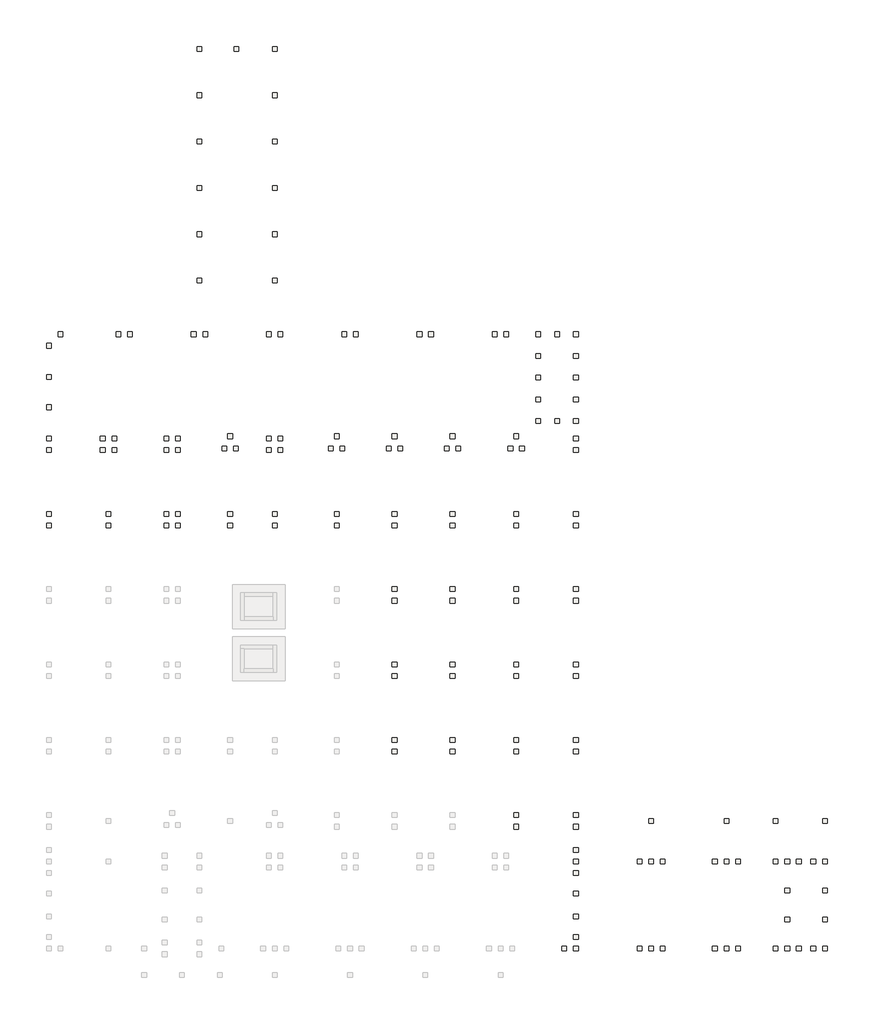
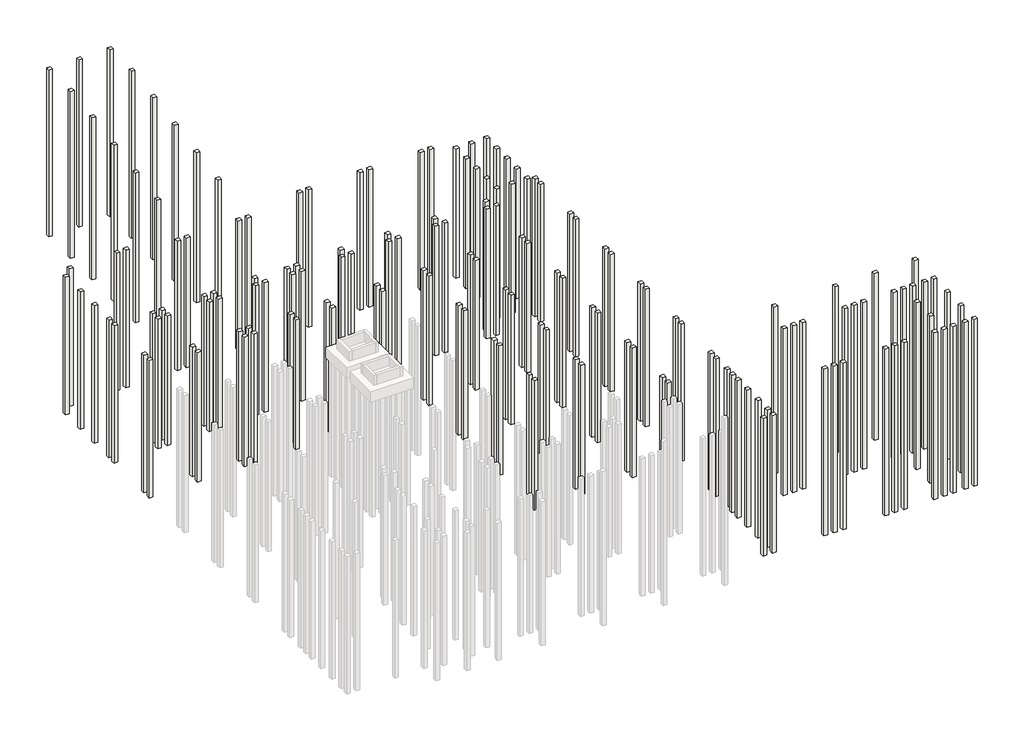
# Not in any storey, part 2 of 2: 160 slabs.
"""IFC4 building model written with IfcOpenShell, lengths in millimetres."""

import ifcopenshell
import ifcopenshell.guid

model = None  # the IFC model being written
_history = None  # IfcOwnerHistory: only IFC2X3 demands one
_inside = {}  # id of a spatial element -> (the spatial element, [elements in it])
_under = {}  # id of a project, library or spatial element -> (it, [spatial elements below it])
_declared = {}  # id of a project -> (the project, [libraries it declares])
_typed = {}  # id of a type object -> (the type object, [elements of that type])
_made_of = {}  # id of a material, layer set ... -> (it, [elements and type objects made of it])


def new_model(schema):
    """Start an empty IFC model of exactly this schema.

    Asked for "IFC4X3", IfcOpenShell would pick the latest addendum, in which some entities
    have other attributes; the version numbers below select the first issue.
    IFC2X3 requires an IfcOwnerHistory on every rooted entity: one is made here for all.
    """
    global model, _history
    if schema == "IFC4X3":
        model = ifcopenshell.file(schema_version=(4, 3, 0, 0))
    else:
        model = ifcopenshell.file(schema=schema)
    _inside.clear()
    _under.clear()
    _declared.clear()
    _typed.clear()
    _made_of.clear()
    _history = None
    if model.schema == "IFC2X3":
        org = make("IfcOrganization", Name="unknown")
        user = make(
            "IfcPersonAndOrganization",
            ThePerson=make("IfcPerson", FamilyName="unknown"),
            TheOrganization=org,
        )
        app = make(
            "IfcApplication",
            ApplicationDeveloper=org,
            Version="unknown",
            ApplicationFullName="unknown",
            ApplicationIdentifier="unknown",
        )
        _history = make(
            "IfcOwnerHistory",
            OwningUser=user,
            OwningApplication=app,
            ChangeAction="ADDED",
            CreationDate=0,
        )
    return model


def make(cls, **values):
    """One entity of the class cls with the attributes given. An attribute that is None is left unset."""
    return model.create_entity(
        cls, **{name: value for name, value in values.items() if value is not None}
    )


def rooted(cls, **values):
    """An entity with a GlobalId (a new one), such as an element, a storey or a relation."""
    return make(cls, GlobalId=ifcopenshell.guid.new(), OwnerHistory=_history, **values)


def si_unit(unit_type, name, prefix=None):
    """IfcSIUnit, for example si_unit("LENGTHUNIT", "METRE", prefix="MILLI")."""
    return make("IfcSIUnit", UnitType=unit_type, Prefix=prefix, Name=name)


def assignment(units):
    """IfcUnitAssignment: the units of a project."""
    return None if units is None else make("IfcUnitAssignment", Units=units)


def point(xyz):
    """IfcCartesianPoint."""
    return None if xyz is None else make("IfcCartesianPoint", Coordinates=xyz)


def direction(xyz):
    """IfcDirection."""
    return None if xyz is None else make("IfcDirection", DirectionRatios=xyz)


def frame(location, z_axis=None, x_axis=None):
    """IfcAxis2Placement3D, a coordinate frame: its origin and axes. An axis left out is left unset."""
    return make(
        "IfcAxis2Placement3D",
        Location=point(location),
        Axis=direction(z_axis),
        RefDirection=direction(x_axis),
    )


def origin():
    """The frame at (0, 0, 0) with its axes left unset."""
    return frame((0.0, 0.0, 0.0))


def place(relative_to, where):
    """IfcLocalPlacement: puts the frame where relative to a parent placement (None: the world)."""
    return make(
        "IfcLocalPlacement", PlacementRelTo=relative_to, RelativePlacement=where
    )


def context(
    kind, dimensions, precision=None, world=None, true_north=None, identifier=None
):
    """IfcGeometricRepresentationContext, for example the 3D "Model" context."""
    return make(
        "IfcGeometricRepresentationContext",
        ContextIdentifier=identifier,
        ContextType=kind,
        CoordinateSpaceDimension=dimensions,
        Precision=precision,
        WorldCoordinateSystem=world,
        TrueNorth=true_north,
    )


def project(units=None, contexts=None):
    """IfcProject with its units and contexts."""
    return rooted(
        "IfcProject",
        Name="project",
        RepresentationContexts=contexts,
        UnitsInContext=assignment(units),
    )


def spatial(cls, under=None, at=None, **own):
    """A site, building, storey or space (cls), placed at a placement, below another one or the project."""
    s = rooted(cls, ObjectPlacement=at, **own)
    if under is not None:
        _under.setdefault(under.id(), (under, []))[1].append(s)
    return s


def polyline(points):
    """IfcPolyline through the points."""
    return make("IfcPolyline", Points=[point(p) for p in points])


def outline(outer, holes=None, kind="AREA"):
    """IfcArbitraryClosedProfileDef: a profile drawn as a closed curve; with holes, ...WithVoids."""
    if holes is None:
        return make("IfcArbitraryClosedProfileDef", ProfileType=kind, OuterCurve=outer)
    return make(
        "IfcArbitraryProfileDefWithVoids",
        ProfileType=kind,
        OuterCurve=outer,
        InnerCurves=holes,
    )


def extrude(swept, where, along, depth):
    """IfcExtrudedAreaSolid: the profile swept, set in the frame where, extruded along a direction by depth."""
    return make(
        "IfcExtrudedAreaSolid",
        SweptArea=swept,
        Position=where,
        ExtrudedDirection=direction(along),
        Depth=depth,
    )


def shape(context_of_items, identifier, shape_type, items):
    """IfcShapeRepresentation: the items that make up one representation, for example the "Body"."""
    return make(
        "IfcShapeRepresentation",
        ContextOfItems=context_of_items,
        RepresentationIdentifier=identifier,
        RepresentationType=shape_type,
        Items=items,
    )


def source(mapping_origin, context_of_items, identifier, shape_type, items):
    """IfcRepresentationMap: a shape defined once, which mapped items show again and again."""
    return make(
        "IfcRepresentationMap",
        MappingOrigin=mapping_origin,
        MappedRepresentation=shape(context_of_items, identifier, shape_type, items),
    )


def transform(
    local_origin,
    x_axis=None,
    y_axis=None,
    z_axis=None,
    scale=None,
    scale2=None,
    scale3=None,
    uniform=True,
):
    """IfcCartesianTransformationOperator3D, or its non-uniform kind. x_axis, y_axis, z_axis: its Axis1, 2, 3."""
    if uniform:
        return make(
            "IfcCartesianTransformationOperator3D",
            Axis1=direction(x_axis),
            Axis2=direction(y_axis),
            LocalOrigin=point(local_origin),
            Scale=scale,
            Axis3=direction(z_axis),
        )
    return make(
        "IfcCartesianTransformationOperator3DnonUniform",
        Axis1=direction(x_axis),
        Axis2=direction(y_axis),
        LocalOrigin=point(local_origin),
        Scale=scale,
        Axis3=direction(z_axis),
        Scale2=scale2,
        Scale3=scale3,
    )


def mapped(mapping_source, mapping_target):
    """IfcMappedItem: shows the shape of a source again, moved by a transform."""
    return make(
        "IfcMappedItem", MappingSource=mapping_source, MappingTarget=mapping_target
    )


def made_of(thing, what):
    """Note that an element or type object is made of a material, layer set ...; save() writes the relation."""
    if what is not None:
        _made_of.setdefault(what.id(), (what, []))[1].append(thing)
    return thing


def element(
    cls,
    number,
    at=None,
    inside=None,
    cuts=None,
    type_object=None,
    material=None,
    context=None,
    identifier="Body",
    shape_type=None,
    held_by="IfcProductDefinitionShape",
    body=None,
    shapes=None,
    **own,
):
    """One element of the class cls, such as IfcWall. Its Tag is "e" and its number.

    at: its placement. inside: the storey or other place that contains it. cuts: it is an
    opening in that element (IfcRelVoidsElement). A single representation is given by context,
    identifier, shape_type and body (its items); several are given by shapes. held_by: the class
    of the entity that holds the representations. save() writes the other relations.
    """
    e = rooted(cls, Tag="e%d" % number, ObjectPlacement=at, **own)
    if body is not None:
        shapes = [shape(context, identifier, shape_type, body)]
    if shapes is not None:
        e.Representation = make(held_by, Representations=shapes)
    if inside is not None:
        _inside.setdefault(inside.id(), (inside, []))[1].append(e)
    if cuts is not None:
        rooted(
            "IfcRelVoidsElement", RelatingBuildingElement=cuts, RelatedOpeningElement=e
        )
    if type_object is not None:
        _typed.setdefault(type_object.id(), (type_object, []))[1].append(e)
    return made_of(e, material)


def aggregate(whole, parts):
    """IfcRelAggregates: a whole, such as a stair, and the parts it consists of."""
    return rooted("IfcRelAggregates", RelatingObject=whole, RelatedObjects=parts)


def save(model, path):
    """Write the relations noted so far, then the file.

    IfcRelAggregates (storeys below a building ...), IfcRelContainedInSpatialStructure (elements
    in a storey), IfcRelDefinesByType, IfcRelAssociatesMaterial and IfcRelDeclares: one each for
    every whole, place, type object, material and project.
    """
    for whole, parts in _under.values():
        aggregate(whole, parts)
    for where, things in _inside.values():
        rooted(
            "IfcRelContainedInSpatialStructure",
            RelatedElements=things,
            RelatingStructure=where,
        )
    for kind, things in _typed.values():
        rooted("IfcRelDefinesByType", RelatedObjects=things, RelatingType=kind)
    for what, things in _made_of.values():
        rooted("IfcRelAssociatesMaterial", RelatedObjects=things, RelatingMaterial=what)
    for by, libraries in _declared.values():
        rooted("IfcRelDeclares", RelatingContext=by, RelatedDefinitions=libraries)
    model.write(path)


def slab_2462c6b3(model_context):
    return source(origin(), model_context, "Body", "SweptSolid", [
        extrude(outline(polyline([(200.0, -200.0), (-200.0, -200.0), (-200.0, 200.0), (200.0, 200.0), (200.0, -200.0)])), frame((0.0, 0.0, -20000.0), z_axis=(0.0, 0.0, 1.0), x_axis=(1.0, 0.0, 0.0)), (0.0, 0.0, 1.0), 14620.0),
    ])


def slab_4eaa82be(model_context):
    return source(origin(), model_context, "Body", "SweptSolid", [
        extrude(outline(polyline([(200.0, -200.0), (-200.0, -200.0), (-200.0, 200.0), (200.0, 200.0), (200.0, -200.0)])), frame((0.0, 0.0, -20000.0), z_axis=(0.0, 0.0, 1.0), x_axis=(1.0, 0.0, 0.0)), (0.0, 0.0, 1.0), 15520.0),
    ])


def slab_c87ae41e(model_context):
    return source(origin(), model_context, "Body", "SweptSolid", [
        extrude(outline(polyline([(200.0, -200.0), (-200.0, -200.0), (-200.0, 200.0), (200.0, 200.0), (200.0, -200.0)])), frame((0.0, 0.0, -20000.0), z_axis=(0.0, 0.0, 1.0), x_axis=(1.0, 0.0, 0.0)), (0.0, 0.0, 1.0), 18830.0),
    ])


def slab_0d914d5e(model_context):
    return source(origin(), model_context, "Body", "SweptSolid", [
        extrude(outline(polyline([(200.0, -200.0), (-200.0, -200.0), (-200.0, 200.0), (200.0, 200.0), (200.0, -200.0)])), frame((0.0, 0.0, -20000.0), z_axis=(0.0, 0.0, 1.0), x_axis=(1.0, 0.0, 0.0)), (0.0, 0.0, 1.0), 18850.0),
    ])


def slab_c32f4c5b(model_context):
    return source(origin(), model_context, "Body", "SweptSolid", [
        extrude(outline(polyline([(200.0, -200.0), (-200.0, -200.0), (-200.0, 200.0), (200.0, 200.0), (200.0, -200.0)])), frame((0.0, 0.0, -20000.0), z_axis=(0.0, 0.0, 1.0), x_axis=(1.0, 0.0, 0.0)), (0.0, 0.0, 1.0), 18290.0),
    ])


def slab_f6128070(model_context):
    return source(origin(), model_context, "Body", "SweptSolid", [
        extrude(outline(polyline([(200.0, -200.0), (-200.0, -200.0), (-200.0, 200.0), (200.0, 200.0), (200.0, -200.0)])), frame((0.0, 0.0, -20000.0), z_axis=(0.0, 0.0, 1.0), x_axis=(1.0, 0.0, 0.0)), (0.0, 0.0, 1.0), 17610.0),
    ])


def slab_f9187350(model_context):
    return source(origin(), model_context, "Body", "SweptSolid", [
        extrude(outline(polyline([(200.0, -200.0), (-200.0, -200.0), (-200.0, 200.0), (200.0, 200.0), (200.0, -200.0)])), frame((0.0, 0.0, -20000.0), z_axis=(0.0, 0.0, 1.0), x_axis=(1.0, 0.0, 0.0)), (0.0, 0.0, 1.0), 16925.0),
    ])


def slab_d279473c(model_context):
    return source(origin(), model_context, "Body", "SweptSolid", [
        extrude(outline(polyline([(200.0, -200.0), (-200.0, -200.0), (-200.0, 200.0), (200.0, 200.0), (200.0, -200.0)])), frame((0.0, 0.0, -20000.0), z_axis=(0.0, 0.0, 1.0), x_axis=(1.0, 0.0, 0.0)), (0.0, 0.0, 1.0), 16250.0),
    ])


model = new_model("IFC4")

# Units and contexts
model_context = context("Model", 3, world=origin())
ifc_project = project(units=[si_unit("LENGTHUNIT", "METRE", prefix="MILLI")], contexts=[model_context])

# Site, building
site = spatial("IfcSite", under=ifc_project)
building = spatial("IfcBuilding", under=site)

# Slabs
placement = place(None, origin())
slab_shape = slab_2462c6b3(model_context)
element("IfcSlab", 1, at=placement, inside=building, context=model_context, shape_type="MappedRepresentation", body=[
    mapped(slab_shape, transform((11650.0, 36500.0, 0.0), x_axis=(1.0, 0.0, 0.0), y_axis=(0.0, 1.0, 0.0), z_axis=(0.0, 0.0, 1.0))),
])
element("IfcSlab", 2, at=placement, inside=building, context=model_context, shape_type="MappedRepresentation", body=[
    mapped(slab_shape, transform((11650.0, 37500.0, 0.0), x_axis=(1.0, 0.0, 0.0), y_axis=(0.0, 1.0, 0.0), z_axis=(0.0, 0.0, 1.0))),
])
element("IfcSlab", 3, at=placement, inside=building, context=model_context, shape_type="MappedRepresentation", body=[
    mapped(slab_shape, transform((22150.0, 36500.0, 0.0), x_axis=(1.0, 0.0, 0.0), y_axis=(0.0, 1.0, 0.0), z_axis=(0.0, 0.0, 1.0))),
])
element("IfcSlab", 4, at=placement, inside=building, context=model_context, shape_type="MappedRepresentation", body=[
    mapped(slab_shape, transform((22150.0, 37500.0, 0.0), x_axis=(1.0, 0.0, 0.0), y_axis=(0.0, 1.0, 0.0), z_axis=(0.0, 0.0, 1.0))),
])
element("IfcSlab", 5, at=placement, inside=building, context=model_context, shape_type="MappedRepresentation", body=[
    mapped(slab_shape, transform((26000.0, 36500.0, 0.0), x_axis=(1.0, 0.0, 0.0), y_axis=(0.0, 1.0, 0.0), z_axis=(0.0, 0.0, 1.0))),
])
element("IfcSlab", 6, at=placement, inside=building, context=model_context, shape_type="MappedRepresentation", body=[
    mapped(slab_shape, transform((26000.0, 37500.0, 0.0), x_axis=(1.0, 0.0, 0.0), y_axis=(0.0, 1.0, 0.0), z_axis=(0.0, 0.0, 1.0))),
])
element("IfcSlab", 7, at=placement, inside=building, context=model_context, shape_type="MappedRepresentation", body=[
    mapped(slab_shape, transform((46850.0, 10500.0, 0.0), x_axis=(1.0, 0.0, 0.0), y_axis=(0.0, 1.0, 0.0), z_axis=(0.0, 0.0, 1.0))),
])
element("IfcSlab", 8, at=placement, inside=building, context=model_context, shape_type="MappedRepresentation", body=[
    mapped(slab_shape, transform((46850.0, 11500.0, 0.0), x_axis=(1.0, 0.0, 0.0), y_axis=(0.0, 1.0, 0.0), z_axis=(0.0, 0.0, 1.0))),
])
element("IfcSlab", 9, at=placement, inside=building, context=model_context, shape_type="MappedRepresentation", body=[
    mapped(slab_shape, transform((17650.0, 36500.0, 0.0), x_axis=(1.0, 0.0, 0.0), y_axis=(0.0, 1.0, 0.0), z_axis=(0.0, 0.0, 1.0))),
])
element("IfcSlab", 10, at=placement, inside=building, context=model_context, shape_type="MappedRepresentation", body=[
    mapped(slab_shape, transform((17650.0, 37500.0, 0.0), x_axis=(1.0, 0.0, 0.0), y_axis=(0.0, 1.0, 0.0), z_axis=(0.0, 0.0, 1.0))),
])
element("IfcSlab", 11, at=placement, inside=building, context=model_context, shape_type="MappedRepresentation", body=[
    mapped(slab_shape, transform((16650.0, 36500.0, 0.0), x_axis=(1.0, 0.0, 0.0), y_axis=(0.0, 1.0, 0.0), z_axis=(0.0, 0.0, 1.0))),
])
element("IfcSlab", 12, at=placement, inside=building, context=model_context, shape_type="MappedRepresentation", body=[
    mapped(slab_shape, transform((16650.0, 37500.0, 0.0), x_axis=(1.0, 0.0, 0.0), y_axis=(0.0, 1.0, 0.0), z_axis=(0.0, 0.0, 1.0))),
])
element("IfcSlab", 13, at=placement, inside=building, context=model_context, shape_type="MappedRepresentation", body=[
    mapped(slab_shape, transform((48755.0, 45500.0, 0.0), x_axis=(1.0, 0.0, 0.0), y_axis=(0.0, 1.0, 0.0), z_axis=(0.0, 0.0, 1.0))),
])
element("IfcSlab", 14, at=placement, inside=building, context=model_context, shape_type="MappedRepresentation", body=[
    mapped(slab_shape, transform((52000.0, 45500.0, 0.0), x_axis=(1.0, 0.0, 0.0), y_axis=(0.0, 1.0, 0.0), z_axis=(0.0, 0.0, 1.0))),
])
element("IfcSlab", 15, at=placement, inside=building, context=model_context, shape_type="MappedRepresentation", body=[
    mapped(slab_shape, transform((52000.0, 53000.0, 0.0), x_axis=(1.0, 0.0, 0.0), y_axis=(0.0, 1.0, 0.0), z_axis=(0.0, 0.0, 1.0))),
])
element("IfcSlab", 16, at=placement, inside=building, context=model_context, shape_type="MappedRepresentation", body=[
    mapped(slab_shape, transform((48755.0, 53000.0, 0.0), x_axis=(1.0, 0.0, 0.0), y_axis=(0.0, 1.0, 0.0), z_axis=(0.0, 0.0, 1.0))),
])
element("IfcSlab", 17, at=placement, inside=building, context=model_context, shape_type="MappedRepresentation", body=[
    mapped(slab_shape, transform((50377.5, 53000.0, 0.0), x_axis=(1.0, 0.0, 0.0), y_axis=(0.0, 1.0, 0.0), z_axis=(0.0, 0.0, 1.0))),
])
element("IfcSlab", 18, at=placement, inside=building, context=model_context, shape_type="MappedRepresentation", body=[
    mapped(slab_shape, transform((50377.5, 45500.0, 0.0), x_axis=(1.0, 0.0, 0.0), y_axis=(0.0, 1.0, 0.0), z_axis=(0.0, 0.0, 1.0))),
])
element("IfcSlab", 19, at=placement, inside=building, context=model_context, shape_type="MappedRepresentation", body=[
    mapped(slab_shape, transform((48755.0, 47375.0, 0.0), x_axis=(1.0, 0.0, 0.0), y_axis=(0.0, 1.0, 0.0), z_axis=(0.0, 0.0, 1.0))),
])
element("IfcSlab", 20, at=placement, inside=building, context=model_context, shape_type="MappedRepresentation", body=[
    mapped(slab_shape, transform((48755.0, 49250.0, 0.0), x_axis=(1.0, 0.0, 0.0), y_axis=(0.0, 1.0, 0.0), z_axis=(0.0, 0.0, 1.0))),
])
element("IfcSlab", 21, at=placement, inside=building, context=model_context, shape_type="MappedRepresentation", body=[
    mapped(slab_shape, transform((48755.0, 51125.0, 0.0), x_axis=(1.0, 0.0, 0.0), y_axis=(0.0, 1.0, 0.0), z_axis=(0.0, 0.0, 1.0))),
])
element("IfcSlab", 22, at=placement, inside=building, context=model_context, shape_type="MappedRepresentation", body=[
    mapped(slab_shape, transform((52000.0, 47375.0, 0.0), x_axis=(1.0, 0.0, 0.0), y_axis=(0.0, 1.0, 0.0), z_axis=(0.0, 0.0, 1.0))),
])
element("IfcSlab", 23, at=placement, inside=building, context=model_context, shape_type="MappedRepresentation", body=[
    mapped(slab_shape, transform((52000.0, 49250.0, 0.0), x_axis=(1.0, 0.0, 0.0), y_axis=(0.0, 1.0, 0.0), z_axis=(0.0, 0.0, 1.0))),
])
element("IfcSlab", 24, at=placement, inside=building, context=model_context, shape_type="MappedRepresentation", body=[
    mapped(slab_shape, transform((52000.0, 51125.0, 0.0), x_axis=(1.0, 0.0, 0.0), y_axis=(0.0, 1.0, 0.0), z_axis=(0.0, 0.0, 1.0))),
])
element("IfcSlab", 25, at=placement, inside=building, context=model_context, shape_type="MappedRepresentation", body=[
    mapped(slab_shape, transform((36350.0, 17000.0, 0.0), x_axis=(1.0, 0.0, 0.0), y_axis=(0.0, 1.0, 0.0), z_axis=(0.0, 0.0, 1.0))),
])
element("IfcSlab", 26, at=placement, inside=building, context=model_context, shape_type="MappedRepresentation", body=[
    mapped(slab_shape, transform((36350.0, 18000.0, 0.0), x_axis=(1.0, 0.0, 0.0), y_axis=(0.0, 1.0, 0.0), z_axis=(0.0, 0.0, 1.0))),
])
element("IfcSlab", 27, at=placement, inside=building, context=model_context, shape_type="MappedRepresentation", body=[
    mapped(slab_shape, transform((41350.0, 17000.0, 0.0), x_axis=(1.0, 0.0, 0.0), y_axis=(0.0, 1.0, 0.0), z_axis=(0.0, 0.0, 1.0))),
])
element("IfcSlab", 28, at=placement, inside=building, context=model_context, shape_type="MappedRepresentation", body=[
    mapped(slab_shape, transform((41350.0, 18000.0, 0.0), x_axis=(1.0, 0.0, 0.0), y_axis=(0.0, 1.0, 0.0), z_axis=(0.0, 0.0, 1.0))),
])
element("IfcSlab", 29, at=placement, inside=building, context=model_context, shape_type="MappedRepresentation", body=[
    mapped(slab_shape, transform((46850.0, 17000.0, 0.0), x_axis=(1.0, 0.0, 0.0), y_axis=(0.0, 1.0, 0.0), z_axis=(0.0, 0.0, 1.0))),
])
element("IfcSlab", 30, at=placement, inside=building, context=model_context, shape_type="MappedRepresentation", body=[
    mapped(slab_shape, transform((46850.0, 18000.0, 0.0), x_axis=(1.0, 0.0, 0.0), y_axis=(0.0, 1.0, 0.0), z_axis=(0.0, 0.0, 1.0))),
])
element("IfcSlab", 31, at=placement, inside=building, context=model_context, shape_type="MappedRepresentation", body=[
    mapped(slab_shape, transform((46850.0, 23500.0, 0.0), x_axis=(1.0, 0.0, 0.0), y_axis=(0.0, 1.0, 0.0), z_axis=(0.0, 0.0, 1.0))),
])
element("IfcSlab", 32, at=placement, inside=building, context=model_context, shape_type="MappedRepresentation", body=[
    mapped(slab_shape, transform((46850.0, 24500.0, 0.0), x_axis=(1.0, 0.0, 0.0), y_axis=(0.0, 1.0, 0.0), z_axis=(0.0, 0.0, 1.0))),
])
element("IfcSlab", 33, at=placement, inside=building, context=model_context, shape_type="MappedRepresentation", body=[
    mapped(slab_shape, transform((41350.0, 23500.0, 0.0), x_axis=(1.0, 0.0, 0.0), y_axis=(0.0, 1.0, 0.0), z_axis=(0.0, 0.0, 1.0))),
])
element("IfcSlab", 34, at=placement, inside=building, context=model_context, shape_type="MappedRepresentation", body=[
    mapped(slab_shape, transform((41350.0, 24500.0, 0.0), x_axis=(1.0, 0.0, 0.0), y_axis=(0.0, 1.0, 0.0), z_axis=(0.0, 0.0, 1.0))),
])
element("IfcSlab", 35, at=placement, inside=building, context=model_context, shape_type="MappedRepresentation", body=[
    mapped(slab_shape, transform((36350.0, 23500.0, 0.0), x_axis=(1.0, 0.0, 0.0), y_axis=(0.0, 1.0, 0.0), z_axis=(0.0, 0.0, 1.0))),
])
element("IfcSlab", 36, at=placement, inside=building, context=model_context, shape_type="MappedRepresentation", body=[
    mapped(slab_shape, transform((36350.0, 24500.0, 0.0), x_axis=(1.0, 0.0, 0.0), y_axis=(0.0, 1.0, 0.0), z_axis=(0.0, 0.0, 1.0))),
])
element("IfcSlab", 37, at=placement, inside=building, context=model_context, shape_type="MappedRepresentation", body=[
    mapped(slab_shape, transform((36350.0, 30000.0, 0.0), x_axis=(1.0, 0.0, 0.0), y_axis=(0.0, 1.0, 0.0), z_axis=(0.0, 0.0, 1.0))),
])
element("IfcSlab", 38, at=placement, inside=building, context=model_context, shape_type="MappedRepresentation", body=[
    mapped(slab_shape, transform((36350.0, 31000.0, 0.0), x_axis=(1.0, 0.0, 0.0), y_axis=(0.0, 1.0, 0.0), z_axis=(0.0, 0.0, 1.0))),
])
element("IfcSlab", 39, at=placement, inside=building, context=model_context, shape_type="MappedRepresentation", body=[
    mapped(slab_shape, transform((41350.0, 30000.0, 0.0), x_axis=(1.0, 0.0, 0.0), y_axis=(0.0, 1.0, 0.0), z_axis=(0.0, 0.0, 1.0))),
])
element("IfcSlab", 40, at=placement, inside=building, context=model_context, shape_type="MappedRepresentation", body=[
    mapped(slab_shape, transform((41350.0, 31000.0, 0.0), x_axis=(1.0, 0.0, 0.0), y_axis=(0.0, 1.0, 0.0), z_axis=(0.0, 0.0, 1.0))),
])
element("IfcSlab", 41, at=placement, inside=building, context=model_context, shape_type="MappedRepresentation", body=[
    mapped(slab_shape, transform((46850.0, 30000.0, 0.0), x_axis=(1.0, 0.0, 0.0), y_axis=(0.0, 1.0, 0.0), z_axis=(0.0, 0.0, 1.0))),
])
element("IfcSlab", 42, at=placement, inside=building, context=model_context, shape_type="MappedRepresentation", body=[
    mapped(slab_shape, transform((46850.0, 31000.0, 0.0), x_axis=(1.0, 0.0, 0.0), y_axis=(0.0, 1.0, 0.0), z_axis=(0.0, 0.0, 1.0))),
])
element("IfcSlab", 43, at=placement, inside=building, context=model_context, shape_type="MappedRepresentation", body=[
    mapped(slab_shape, transform((46850.0, 36500.0, 0.0), x_axis=(1.0, 0.0, 0.0), y_axis=(0.0, 1.0, 0.0), z_axis=(0.0, 0.0, 1.0))),
])
element("IfcSlab", 44, at=placement, inside=building, context=model_context, shape_type="MappedRepresentation", body=[
    mapped(slab_shape, transform((46850.0, 37500.0, 0.0), x_axis=(1.0, 0.0, 0.0), y_axis=(0.0, 1.0, 0.0), z_axis=(0.0, 0.0, 1.0))),
])
element("IfcSlab", 45, at=placement, inside=building, context=model_context, shape_type="MappedRepresentation", body=[
    mapped(slab_shape, transform((41350.0, 36500.0, 0.0), x_axis=(1.0, 0.0, 0.0), y_axis=(0.0, 1.0, 0.0), z_axis=(0.0, 0.0, 1.0))),
])
element("IfcSlab", 46, at=placement, inside=building, context=model_context, shape_type="MappedRepresentation", body=[
    mapped(slab_shape, transform((41350.0, 37500.0, 0.0), x_axis=(1.0, 0.0, 0.0), y_axis=(0.0, 1.0, 0.0), z_axis=(0.0, 0.0, 1.0))),
])
element("IfcSlab", 47, at=placement, inside=building, context=model_context, shape_type="MappedRepresentation", body=[
    mapped(slab_shape, transform((36350.0, 36500.0, 0.0), x_axis=(1.0, 0.0, 0.0), y_axis=(0.0, 1.0, 0.0), z_axis=(0.0, 0.0, 1.0))),
])
element("IfcSlab", 48, at=placement, inside=building, context=model_context, shape_type="MappedRepresentation", body=[
    mapped(slab_shape, transform((36350.0, 37500.0, 0.0), x_axis=(1.0, 0.0, 0.0), y_axis=(0.0, 1.0, 0.0), z_axis=(0.0, 0.0, 1.0))),
])
element("IfcSlab", 49, at=placement, inside=building, context=model_context, shape_type="MappedRepresentation", body=[
    mapped(slab_shape, transform((31350.0, 36500.0, 0.0), x_axis=(1.0, 0.0, 0.0), y_axis=(0.0, 1.0, 0.0), z_axis=(0.0, 0.0, 1.0))),
])
element("IfcSlab", 50, at=placement, inside=building, context=model_context, shape_type="MappedRepresentation", body=[
    mapped(slab_shape, transform((31350.0, 37500.0, 0.0), x_axis=(1.0, 0.0, 0.0), y_axis=(0.0, 1.0, 0.0), z_axis=(0.0, 0.0, 1.0))),
])
element("IfcSlab", 51, at=placement, inside=building, context=model_context, shape_type="MappedRepresentation", body=[
    mapped(slab_shape, transform((12150.0, 43000.0, 0.0), x_axis=(1.0, 0.0, 0.0), y_axis=(0.0, 1.0, 0.0), z_axis=(0.0, 0.0, 1.0))),
])
element("IfcSlab", 52, at=placement, inside=building, context=model_context, shape_type="MappedRepresentation", body=[
    mapped(slab_shape, transform((12150.0, 44000.0, 0.0), x_axis=(1.0, 0.0, 0.0), y_axis=(0.0, 1.0, 0.0), z_axis=(0.0, 0.0, 1.0))),
])
element("IfcSlab", 53, at=placement, inside=building, context=model_context, shape_type="MappedRepresentation", body=[
    mapped(slab_shape, transform((11150.0, 43000.0, 0.0), x_axis=(1.0, 0.0, 0.0), y_axis=(0.0, 1.0, 0.0), z_axis=(0.0, 0.0, 1.0))),
])
element("IfcSlab", 54, at=placement, inside=building, context=model_context, shape_type="MappedRepresentation", body=[
    mapped(slab_shape, transform((11150.0, 44000.0, 0.0), x_axis=(1.0, 0.0, 0.0), y_axis=(0.0, 1.0, 0.0), z_axis=(0.0, 0.0, 1.0))),
])
element("IfcSlab", 55, at=placement, inside=building, context=model_context, shape_type="MappedRepresentation", body=[
    mapped(slab_shape, transform((17650.0, 43000.0, 0.0), x_axis=(1.0, 0.0, 0.0), y_axis=(0.0, 1.0, 0.0), z_axis=(0.0, 0.0, 1.0))),
])
element("IfcSlab", 56, at=placement, inside=building, context=model_context, shape_type="MappedRepresentation", body=[
    mapped(slab_shape, transform((17650.0, 44000.0, 0.0), x_axis=(1.0, 0.0, 0.0), y_axis=(0.0, 1.0, 0.0), z_axis=(0.0, 0.0, 1.0))),
])
element("IfcSlab", 57, at=placement, inside=building, context=model_context, shape_type="MappedRepresentation", body=[
    mapped(slab_shape, transform((16650.0, 43000.0, 0.0), x_axis=(1.0, 0.0, 0.0), y_axis=(0.0, 1.0, 0.0), z_axis=(0.0, 0.0, 1.0))),
])
element("IfcSlab", 58, at=placement, inside=building, context=model_context, shape_type="MappedRepresentation", body=[
    mapped(slab_shape, transform((16650.0, 44000.0, 0.0), x_axis=(1.0, 0.0, 0.0), y_axis=(0.0, 1.0, 0.0), z_axis=(0.0, 0.0, 1.0))),
])
element("IfcSlab", 59, at=placement, inside=building, context=model_context, shape_type="MappedRepresentation", body=[
    mapped(slab_shape, transform((21650.0, 43150.0, 0.0), x_axis=(1.0, 0.0, 0.0), y_axis=(0.0, 1.0, 0.0), z_axis=(0.0, 0.0, 1.0))),
])
element("IfcSlab", 60, at=placement, inside=building, context=model_context, shape_type="MappedRepresentation", body=[
    mapped(slab_shape, transform((22650.0, 43150.0, 0.0), x_axis=(1.0, 0.0, 0.0), y_axis=(0.0, 1.0, 0.0), z_axis=(0.0, 0.0, 1.0))),
])
element("IfcSlab", 61, at=placement, inside=building, context=model_context, shape_type="MappedRepresentation", body=[
    mapped(slab_shape, transform((22150.0, 44200.0, 0.0), x_axis=(1.0, 0.0, 0.0), y_axis=(0.0, 1.0, 0.0), z_axis=(0.0, 0.0, 1.0))),
])
element("IfcSlab", 62, at=placement, inside=building, context=model_context, shape_type="MappedRepresentation", body=[
    mapped(slab_shape, transform((26500.0, 43000.0, 0.0), x_axis=(1.0, 0.0, 0.0), y_axis=(0.0, 1.0, 0.0), z_axis=(0.0, 0.0, 1.0))),
])
element("IfcSlab", 63, at=placement, inside=building, context=model_context, shape_type="MappedRepresentation", body=[
    mapped(slab_shape, transform((26500.0, 44000.0, 0.0), x_axis=(1.0, 0.0, 0.0), y_axis=(0.0, 1.0, 0.0), z_axis=(0.0, 0.0, 1.0))),
])
element("IfcSlab", 64, at=placement, inside=building, context=model_context, shape_type="MappedRepresentation", body=[
    mapped(slab_shape, transform((25500.0, 43000.0, 0.0), x_axis=(1.0, 0.0, 0.0), y_axis=(0.0, 1.0, 0.0), z_axis=(0.0, 0.0, 1.0))),
])
element("IfcSlab", 65, at=placement, inside=building, context=model_context, shape_type="MappedRepresentation", body=[
    mapped(slab_shape, transform((25500.0, 44000.0, 0.0), x_axis=(1.0, 0.0, 0.0), y_axis=(0.0, 1.0, 0.0), z_axis=(0.0, 0.0, 1.0))),
])
element("IfcSlab", 66, at=placement, inside=building, context=model_context, shape_type="MappedRepresentation", body=[
    mapped(slab_shape, transform((30850.0, 43150.0, 0.0), x_axis=(1.0, 0.0, 0.0), y_axis=(0.0, 1.0, 0.0), z_axis=(0.0, 0.0, 1.0))),
])
element("IfcSlab", 67, at=placement, inside=building, context=model_context, shape_type="MappedRepresentation", body=[
    mapped(slab_shape, transform((31850.0, 43150.0, 0.0), x_axis=(1.0, 0.0, 0.0), y_axis=(0.0, 1.0, 0.0), z_axis=(0.0, 0.0, 1.0))),
])
element("IfcSlab", 68, at=placement, inside=building, context=model_context, shape_type="MappedRepresentation", body=[
    mapped(slab_shape, transform((31350.0, 44200.0, 0.0), x_axis=(1.0, 0.0, 0.0), y_axis=(0.0, 1.0, 0.0), z_axis=(0.0, 0.0, 1.0))),
])
element("IfcSlab", 69, at=placement, inside=building, context=model_context, shape_type="MappedRepresentation", body=[
    mapped(slab_shape, transform((35850.0, 43150.0, 0.0), x_axis=(1.0, 0.0, 0.0), y_axis=(0.0, 1.0, 0.0), z_axis=(0.0, 0.0, 1.0))),
])
element("IfcSlab", 70, at=placement, inside=building, context=model_context, shape_type="MappedRepresentation", body=[
    mapped(slab_shape, transform((36850.0, 43150.0, 0.0), x_axis=(1.0, 0.0, 0.0), y_axis=(0.0, 1.0, 0.0), z_axis=(0.0, 0.0, 1.0))),
])
element("IfcSlab", 71, at=placement, inside=building, context=model_context, shape_type="MappedRepresentation", body=[
    mapped(slab_shape, transform((36350.0, 44200.0, 0.0), x_axis=(1.0, 0.0, 0.0), y_axis=(0.0, 1.0, 0.0), z_axis=(0.0, 0.0, 1.0))),
])
element("IfcSlab", 72, at=placement, inside=building, context=model_context, shape_type="MappedRepresentation", body=[
    mapped(slab_shape, transform((40850.0, 43150.0, 0.0), x_axis=(1.0, 0.0, 0.0), y_axis=(0.0, 1.0, 0.0), z_axis=(0.0, 0.0, 1.0))),
])
element("IfcSlab", 73, at=placement, inside=building, context=model_context, shape_type="MappedRepresentation", body=[
    mapped(slab_shape, transform((41850.0, 43150.0, 0.0), x_axis=(1.0, 0.0, 0.0), y_axis=(0.0, 1.0, 0.0), z_axis=(0.0, 0.0, 1.0))),
])
element("IfcSlab", 74, at=placement, inside=building, context=model_context, shape_type="MappedRepresentation", body=[
    mapped(slab_shape, transform((41350.0, 44200.0, 0.0), x_axis=(1.0, 0.0, 0.0), y_axis=(0.0, 1.0, 0.0), z_axis=(0.0, 0.0, 1.0))),
])
element("IfcSlab", 75, at=placement, inside=building, context=model_context, shape_type="MappedRepresentation", body=[
    mapped(slab_shape, transform((46350.0, 43150.0, 0.0), x_axis=(1.0, 0.0, 0.0), y_axis=(0.0, 1.0, 0.0), z_axis=(0.0, 0.0, 1.0))),
])
element("IfcSlab", 76, at=placement, inside=building, context=model_context, shape_type="MappedRepresentation", body=[
    mapped(slab_shape, transform((47350.0, 43150.0, 0.0), x_axis=(1.0, 0.0, 0.0), y_axis=(0.0, 1.0, 0.0), z_axis=(0.0, 0.0, 1.0))),
])
element("IfcSlab", 77, at=placement, inside=building, context=model_context, shape_type="MappedRepresentation", body=[
    mapped(slab_shape, transform((46850.0, 44200.0, 0.0), x_axis=(1.0, 0.0, 0.0), y_axis=(0.0, 1.0, 0.0), z_axis=(0.0, 0.0, 1.0))),
])
element("IfcSlab", 78, at=placement, inside=building, context=model_context, shape_type="MappedRepresentation", body=[
    mapped(slab_shape, transform((25500.0, 53000.0, 0.0), x_axis=(1.0, 0.0, 0.0), y_axis=(0.0, 1.0, 0.0), z_axis=(0.0, 0.0, 1.0))),
])
element("IfcSlab", 79, at=placement, inside=building, context=model_context, shape_type="MappedRepresentation", body=[
    mapped(slab_shape, transform((26500.0, 53000.0, 0.0), x_axis=(1.0, 0.0, 0.0), y_axis=(0.0, 1.0, 0.0), z_axis=(0.0, 0.0, 1.0))),
])
element("IfcSlab", 80, at=placement, inside=building, context=model_context, shape_type="MappedRepresentation", body=[
    mapped(slab_shape, transform((19000.0, 53000.0, 0.0), x_axis=(1.0, 0.0, 0.0), y_axis=(0.0, 1.0, 0.0), z_axis=(0.0, 0.0, 1.0))),
])
element("IfcSlab", 81, at=placement, inside=building, context=model_context, shape_type="MappedRepresentation", body=[
    mapped(slab_shape, transform((20000.0, 53000.0, 0.0), x_axis=(1.0, 0.0, 0.0), y_axis=(0.0, 1.0, 0.0), z_axis=(0.0, 0.0, 1.0))),
])
slab_2_shape = slab_4eaa82be(model_context)
element("IfcSlab", 82, at=placement, inside=building, context=model_context, shape_type="MappedRepresentation", body=[
    mapped(slab_2_shape, transform((7500.0, 53000.0, 0.0), x_axis=(1.0, 0.0, 0.0), y_axis=(0.0, 1.0, 0.0), z_axis=(0.0, 0.0, 1.0))),
])
element("IfcSlab", 83, at=placement, inside=building, context=model_context, shape_type="MappedRepresentation", body=[
    mapped(slab_2_shape, transform((6500.0, 52000.0, 0.0), x_axis=(1.0, 0.0, 0.0), y_axis=(0.0, 1.0, 0.0), z_axis=(0.0, 0.0, 1.0))),
])
element("IfcSlab", 84, at=placement, inside=building, context=model_context, shape_type="MappedRepresentation", body=[
    mapped(slab_2_shape, transform((6500.0, 43000.0, 0.0), x_axis=(1.0, 0.0, 0.0), y_axis=(0.0, 1.0, 0.0), z_axis=(0.0, 0.0, 1.0))),
])
element("IfcSlab", 85, at=placement, inside=building, context=model_context, shape_type="MappedRepresentation", body=[
    mapped(slab_2_shape, transform((6500.0, 44000.0, 0.0), x_axis=(1.0, 0.0, 0.0), y_axis=(0.0, 1.0, 0.0), z_axis=(0.0, 0.0, 1.0))),
])
element("IfcSlab", 86, at=placement, inside=building, context=model_context, shape_type="MappedRepresentation", body=[
    mapped(slab_2_shape, transform((6500.0, 46700.0, 0.0), x_axis=(1.0, 0.0, 0.0), y_axis=(0.0, 1.0, 0.0), z_axis=(0.0, 0.0, 1.0))),
])
element("IfcSlab", 87, at=placement, inside=building, context=model_context, shape_type="MappedRepresentation", body=[
    mapped(slab_2_shape, transform((52000.0, 43000.0, 0.0), x_axis=(1.0, 0.0, 0.0), y_axis=(0.0, 1.0, 0.0), z_axis=(0.0, 0.0, 1.0))),
])
element("IfcSlab", 88, at=placement, inside=building, context=model_context, shape_type="MappedRepresentation", body=[
    mapped(slab_2_shape, transform((52000.0, 44000.0, 0.0), x_axis=(1.0, 0.0, 0.0), y_axis=(0.0, 1.0, 0.0), z_axis=(0.0, 0.0, 1.0))),
])
element("IfcSlab", 89, at=placement, inside=building, context=model_context, shape_type="MappedRepresentation", body=[
    mapped(slab_2_shape, transform((51000.0, 0.0, 0.0), x_axis=(1.0, 0.0, 0.0), y_axis=(0.0, 1.0, 0.0), z_axis=(0.0, 0.0, 1.0))),
])
element("IfcSlab", 90, at=placement, inside=building, context=model_context, shape_type="MappedRepresentation", body=[
    mapped(slab_2_shape, transform((52000.0, 0.0, 0.0), x_axis=(1.0, 0.0, 0.0), y_axis=(0.0, 1.0, 0.0), z_axis=(0.0, 0.0, 1.0))),
])
element("IfcSlab", 91, at=placement, inside=building, context=model_context, shape_type="MappedRepresentation", body=[
    mapped(slab_2_shape, transform((52000.0, 1000.0, 0.0), x_axis=(1.0, 0.0, 0.0), y_axis=(0.0, 1.0, 0.0), z_axis=(0.0, 0.0, 1.0))),
])
element("IfcSlab", 92, at=placement, inside=building, context=model_context, shape_type="MappedRepresentation", body=[
    mapped(slab_2_shape, transform((52000.0, 2750.0, 0.0), x_axis=(1.0, 0.0, 0.0), y_axis=(0.0, 1.0, 0.0), z_axis=(0.0, 0.0, 1.0))),
])
element("IfcSlab", 93, at=placement, inside=building, context=model_context, shape_type="MappedRepresentation", body=[
    mapped(slab_2_shape, transform((52000.0, 6500.0, 0.0), x_axis=(1.0, 0.0, 0.0), y_axis=(0.0, 1.0, 0.0), z_axis=(0.0, 0.0, 1.0))),
])
element("IfcSlab", 94, at=placement, inside=building, context=model_context, shape_type="MappedRepresentation", body=[
    mapped(slab_2_shape, transform((52000.0, 7500.0, 0.0), x_axis=(1.0, 0.0, 0.0), y_axis=(0.0, 1.0, 0.0), z_axis=(0.0, 0.0, 1.0))),
])
element("IfcSlab", 95, at=placement, inside=building, context=model_context, shape_type="MappedRepresentation", body=[
    mapped(slab_2_shape, transform((52000.0, 8500.0, 0.0), x_axis=(1.0, 0.0, 0.0), y_axis=(0.0, 1.0, 0.0), z_axis=(0.0, 0.0, 1.0))),
])
element("IfcSlab", 96, at=placement, inside=building, context=model_context, shape_type="MappedRepresentation", body=[
    mapped(slab_2_shape, transform((52000.0, 4750.0, 0.0), x_axis=(1.0, 0.0, 0.0), y_axis=(0.0, 1.0, 0.0), z_axis=(0.0, 0.0, 1.0))),
])
element("IfcSlab", 97, at=placement, inside=building, context=model_context, shape_type="MappedRepresentation", body=[
    mapped(slab_2_shape, transform((52000.0, 10500.0, 0.0), x_axis=(1.0, 0.0, 0.0), y_axis=(0.0, 1.0, 0.0), z_axis=(0.0, 0.0, 1.0))),
])
element("IfcSlab", 98, at=placement, inside=building, context=model_context, shape_type="MappedRepresentation", body=[
    mapped(slab_2_shape, transform((52000.0, 11500.0, 0.0), x_axis=(1.0, 0.0, 0.0), y_axis=(0.0, 1.0, 0.0), z_axis=(0.0, 0.0, 1.0))),
])
element("IfcSlab", 99, at=placement, inside=building, context=model_context, shape_type="MappedRepresentation", body=[
    mapped(slab_2_shape, transform((6500.0, 36500.0, 0.0), x_axis=(1.0, 0.0, 0.0), y_axis=(0.0, 1.0, 0.0), z_axis=(0.0, 0.0, 1.0))),
])
element("IfcSlab", 100, at=placement, inside=building, context=model_context, shape_type="MappedRepresentation", body=[
    mapped(slab_2_shape, transform((6500.0, 37500.0, 0.0), x_axis=(1.0, 0.0, 0.0), y_axis=(0.0, 1.0, 0.0), z_axis=(0.0, 0.0, 1.0))),
])
element("IfcSlab", 101, at=placement, inside=building, context=model_context, shape_type="MappedRepresentation", body=[
    mapped(slab_2_shape, transform((52000.0, 17000.0, 0.0), x_axis=(1.0, 0.0, 0.0), y_axis=(0.0, 1.0, 0.0), z_axis=(0.0, 0.0, 1.0))),
])
element("IfcSlab", 102, at=placement, inside=building, context=model_context, shape_type="MappedRepresentation", body=[
    mapped(slab_2_shape, transform((52000.0, 18000.0, 0.0), x_axis=(1.0, 0.0, 0.0), y_axis=(0.0, 1.0, 0.0), z_axis=(0.0, 0.0, 1.0))),
])
element("IfcSlab", 103, at=placement, inside=building, context=model_context, shape_type="MappedRepresentation", body=[
    mapped(slab_2_shape, transform((52000.0, 23500.0, 0.0), x_axis=(1.0, 0.0, 0.0), y_axis=(0.0, 1.0, 0.0), z_axis=(0.0, 0.0, 1.0))),
])
element("IfcSlab", 104, at=placement, inside=building, context=model_context, shape_type="MappedRepresentation", body=[
    mapped(slab_2_shape, transform((52000.0, 24500.0, 0.0), x_axis=(1.0, 0.0, 0.0), y_axis=(0.0, 1.0, 0.0), z_axis=(0.0, 0.0, 1.0))),
])
element("IfcSlab", 105, at=placement, inside=building, context=model_context, shape_type="MappedRepresentation", body=[
    mapped(slab_2_shape, transform((52000.0, 30000.0, 0.0), x_axis=(1.0, 0.0, 0.0), y_axis=(0.0, 1.0, 0.0), z_axis=(0.0, 0.0, 1.0))),
])
element("IfcSlab", 106, at=placement, inside=building, context=model_context, shape_type="MappedRepresentation", body=[
    mapped(slab_2_shape, transform((52000.0, 31000.0, 0.0), x_axis=(1.0, 0.0, 0.0), y_axis=(0.0, 1.0, 0.0), z_axis=(0.0, 0.0, 1.0))),
])
element("IfcSlab", 107, at=placement, inside=building, context=model_context, shape_type="MappedRepresentation", body=[
    mapped(slab_2_shape, transform((52000.0, 36500.0, 0.0), x_axis=(1.0, 0.0, 0.0), y_axis=(0.0, 1.0, 0.0), z_axis=(0.0, 0.0, 1.0))),
])
element("IfcSlab", 108, at=placement, inside=building, context=model_context, shape_type="MappedRepresentation", body=[
    mapped(slab_2_shape, transform((52000.0, 37500.0, 0.0), x_axis=(1.0, 0.0, 0.0), y_axis=(0.0, 1.0, 0.0), z_axis=(0.0, 0.0, 1.0))),
])
element("IfcSlab", 109, at=placement, inside=building, context=model_context, shape_type="MappedRepresentation", body=[
    mapped(slab_2_shape, transform((46000.0, 53000.0, 0.0), x_axis=(1.0, 0.0, 0.0), y_axis=(0.0, 1.0, 0.0), z_axis=(0.0, 0.0, 1.0))),
])
element("IfcSlab", 110, at=placement, inside=building, context=model_context, shape_type="MappedRepresentation", body=[
    mapped(slab_2_shape, transform((45000.0, 53000.0, 0.0), x_axis=(1.0, 0.0, 0.0), y_axis=(0.0, 1.0, 0.0), z_axis=(0.0, 0.0, 1.0))),
])
element("IfcSlab", 111, at=placement, inside=building, context=model_context, shape_type="MappedRepresentation", body=[
    mapped(slab_2_shape, transform((39500.0, 53000.0, 0.0), x_axis=(1.0, 0.0, 0.0), y_axis=(0.0, 1.0, 0.0), z_axis=(0.0, 0.0, 1.0))),
])
element("IfcSlab", 112, at=placement, inside=building, context=model_context, shape_type="MappedRepresentation", body=[
    mapped(slab_2_shape, transform((38500.0, 53000.0, 0.0), x_axis=(1.0, 0.0, 0.0), y_axis=(0.0, 1.0, 0.0), z_axis=(0.0, 0.0, 1.0))),
])
element("IfcSlab", 113, at=placement, inside=building, context=model_context, shape_type="MappedRepresentation", body=[
    mapped(slab_2_shape, transform((33000.0, 53000.0, 0.0), x_axis=(1.0, 0.0, 0.0), y_axis=(0.0, 1.0, 0.0), z_axis=(0.0, 0.0, 1.0))),
])
element("IfcSlab", 114, at=placement, inside=building, context=model_context, shape_type="MappedRepresentation", body=[
    mapped(slab_2_shape, transform((32000.0, 53000.0, 0.0), x_axis=(1.0, 0.0, 0.0), y_axis=(0.0, 1.0, 0.0), z_axis=(0.0, 0.0, 1.0))),
])
element("IfcSlab", 115, at=placement, inside=building, context=model_context, shape_type="MappedRepresentation", body=[
    mapped(slab_2_shape, transform((6500.0, 49300.0, 0.0), x_axis=(1.0, 0.0, 0.0), y_axis=(0.0, 1.0, 0.0), z_axis=(0.0, 0.0, 1.0))),
])
element("IfcSlab", 116, at=placement, inside=building, context=model_context, shape_type="MappedRepresentation", body=[
    mapped(slab_2_shape, transform((13500.0, 53000.0, 0.0), x_axis=(1.0, 0.0, 0.0), y_axis=(0.0, 1.0, 0.0), z_axis=(0.0, 0.0, 1.0))),
])
element("IfcSlab", 117, at=placement, inside=building, context=model_context, shape_type="MappedRepresentation", body=[
    mapped(slab_2_shape, transform((12500.0, 53000.0, 0.0), x_axis=(1.0, 0.0, 0.0), y_axis=(0.0, 1.0, 0.0), z_axis=(0.0, 0.0, 1.0))),
])
slab_3_shape = slab_c87ae41e(model_context)
element("IfcSlab", 118, at=placement, inside=building, context=model_context, shape_type="MappedRepresentation", body=[
    mapped(slab_3_shape, transform((57500.0, 7500.0, 0.0), x_axis=(1.0, 0.0, 0.0), y_axis=(0.0, 1.0, 0.0), z_axis=(0.0, 0.0, 1.0))),
])
element("IfcSlab", 119, at=placement, inside=building, context=model_context, shape_type="MappedRepresentation", body=[
    mapped(slab_3_shape, transform((58500.0, 7500.0, 0.0), x_axis=(-1.0, 0.0, 0.0), y_axis=(0.0, -1.0, 0.0), z_axis=(0.0, 0.0, 1.0))),
])
element("IfcSlab", 120, at=placement, inside=building, context=model_context, shape_type="MappedRepresentation", body=[
    mapped(slab_3_shape, transform((59500.0, 7500.0, 0.0), x_axis=(-1.0, 0.0, 0.0), y_axis=(0.0, -1.0, 0.0), z_axis=(0.0, 0.0, 1.0))),
])
element("IfcSlab", 121, at=placement, inside=building, context=model_context, shape_type="MappedRepresentation", body=[
    mapped(slab_3_shape, transform((64000.0, 7500.0, 0.0), x_axis=(1.0, 0.0, 0.0), y_axis=(0.0, 1.0, 0.0), z_axis=(0.0, 0.0, 1.0))),
])
element("IfcSlab", 122, at=placement, inside=building, context=model_context, shape_type="MappedRepresentation", body=[
    mapped(slab_3_shape, transform((65000.0, 7500.0, 0.0), x_axis=(1.0, 0.0, 0.0), y_axis=(0.0, 1.0, 0.0), z_axis=(0.0, 0.0, 1.0))),
])
element("IfcSlab", 123, at=placement, inside=building, context=model_context, shape_type="MappedRepresentation", body=[
    mapped(slab_3_shape, transform((66000.0, 7500.0, 0.0), x_axis=(1.0, 0.0, 0.0), y_axis=(0.0, 1.0, 0.0), z_axis=(0.0, 0.0, 1.0))),
])
element("IfcSlab", 124, at=placement, inside=building, context=model_context, shape_type="MappedRepresentation", body=[
    mapped(slab_3_shape, transform((57500.0, 0.0, 0.0), x_axis=(1.0, 0.0, 0.0), y_axis=(0.0, 1.0, 0.0), z_axis=(0.0, 0.0, 1.0))),
])
element("IfcSlab", 125, at=placement, inside=building, context=model_context, shape_type="MappedRepresentation", body=[
    mapped(slab_3_shape, transform((58500.0, 0.0, 0.0), x_axis=(1.0, 0.0, 0.0), y_axis=(0.0, 1.0, 0.0), z_axis=(0.0, 0.0, 1.0))),
])
element("IfcSlab", 126, at=placement, inside=building, context=model_context, shape_type="MappedRepresentation", body=[
    mapped(slab_3_shape, transform((59500.0, 0.0, 0.0), x_axis=(1.0, 0.0, 0.0), y_axis=(0.0, 1.0, 0.0), z_axis=(0.0, 0.0, 1.0))),
])
element("IfcSlab", 127, at=placement, inside=building, context=model_context, shape_type="MappedRepresentation", body=[
    mapped(slab_3_shape, transform((64000.0, 0.0, 0.0), x_axis=(1.0, 0.0, 0.0), y_axis=(0.0, 1.0, 0.0), z_axis=(0.0, 0.0, 1.0))),
])
element("IfcSlab", 128, at=placement, inside=building, context=model_context, shape_type="MappedRepresentation", body=[
    mapped(slab_3_shape, transform((65000.0, 0.0, 0.0), x_axis=(1.0, 0.0, 0.0), y_axis=(0.0, 1.0, 0.0), z_axis=(0.0, 0.0, 1.0))),
])
element("IfcSlab", 129, at=placement, inside=building, context=model_context, shape_type="MappedRepresentation", body=[
    mapped(slab_3_shape, transform((66000.0, 0.0, 0.0), x_axis=(1.0, 0.0, 0.0), y_axis=(0.0, 1.0, 0.0), z_axis=(0.0, 0.0, 1.0))),
])
element("IfcSlab", 130, at=placement, inside=building, context=model_context, shape_type="MappedRepresentation", body=[
    mapped(slab_3_shape, transform((70250.0, 0.0, 0.0), x_axis=(1.0, 0.0, 0.0), y_axis=(0.0, 1.0, 0.0), z_axis=(0.0, 0.0, 1.0))),
])
element("IfcSlab", 131, at=placement, inside=building, context=model_context, shape_type="MappedRepresentation", body=[
    mapped(slab_3_shape, transform((71250.0, 0.0, 0.0), x_axis=(1.0, 0.0, 0.0), y_axis=(0.0, 1.0, 0.0), z_axis=(0.0, 0.0, 1.0))),
])
element("IfcSlab", 132, at=placement, inside=building, context=model_context, shape_type="MappedRepresentation", body=[
    mapped(slab_3_shape, transform((73500.0, 0.0, 0.0), x_axis=(1.0, 0.0, 0.0), y_axis=(0.0, 1.0, 0.0), z_axis=(0.0, 0.0, 1.0))),
])
element("IfcSlab", 133, at=placement, inside=building, context=model_context, shape_type="MappedRepresentation", body=[
    mapped(slab_3_shape, transform((70250.0, 7500.0, 0.0), x_axis=(1.0, 0.0, 0.0), y_axis=(0.0, 1.0, 0.0), z_axis=(0.0, 0.0, 1.0))),
])
element("IfcSlab", 134, at=placement, inside=building, context=model_context, shape_type="MappedRepresentation", body=[
    mapped(slab_3_shape, transform((71250.0, 7500.0, 0.0), x_axis=(1.0, 0.0, 0.0), y_axis=(0.0, 1.0, 0.0), z_axis=(0.0, 0.0, 1.0))),
])
element("IfcSlab", 135, at=placement, inside=building, context=model_context, shape_type="MappedRepresentation", body=[
    mapped(slab_3_shape, transform((73500.0, 7500.0, 0.0), x_axis=(1.0, 0.0, 0.0), y_axis=(0.0, 1.0, 0.0), z_axis=(0.0, 0.0, 1.0))),
])
element("IfcSlab", 136, at=placement, inside=building, context=model_context, shape_type="MappedRepresentation", body=[
    mapped(slab_3_shape, transform((70250.0, 5000.0, 0.0), x_axis=(1.0, 0.0, 0.0), y_axis=(0.0, 1.0, 0.0), z_axis=(0.0, 0.0, 1.0))),
])
element("IfcSlab", 137, at=placement, inside=building, context=model_context, shape_type="MappedRepresentation", body=[
    mapped(slab_3_shape, transform((70250.0, 2500.0, 0.0), x_axis=(1.0, 0.0, 0.0), y_axis=(0.0, 1.0, 0.0), z_axis=(0.0, 0.0, 1.0))),
])
element("IfcSlab", 138, at=placement, inside=building, context=model_context, shape_type="MappedRepresentation", body=[
    mapped(slab_3_shape, transform((73500.0, 5000.0, 0.0), x_axis=(1.0, 0.0, 0.0), y_axis=(0.0, 1.0, 0.0), z_axis=(0.0, 0.0, 1.0))),
])
element("IfcSlab", 139, at=placement, inside=building, context=model_context, shape_type="MappedRepresentation", body=[
    mapped(slab_3_shape, transform((73500.0, 2500.0, 0.0), x_axis=(1.0, 0.0, 0.0), y_axis=(0.0, 1.0, 0.0), z_axis=(0.0, 0.0, 1.0))),
])
element("IfcSlab", 140, at=placement, inside=building, context=model_context, shape_type="MappedRepresentation", body=[
    mapped(slab_3_shape, transform((69250.0, 0.0, 0.0), x_axis=(1.0, 0.0, 0.0), y_axis=(0.0, 1.0, 0.0), z_axis=(0.0, 0.0, 1.0))),
])
element("IfcSlab", 141, at=placement, inside=building, context=model_context, shape_type="MappedRepresentation", body=[
    mapped(slab_3_shape, transform((69250.0, 7500.0, 0.0), x_axis=(1.0, 0.0, 0.0), y_axis=(0.0, 1.0, 0.0), z_axis=(0.0, 0.0, 1.0))),
])
element("IfcSlab", 142, at=placement, inside=building, context=model_context, shape_type="MappedRepresentation", body=[
    mapped(slab_3_shape, transform((72500.0, 0.0, 0.0), x_axis=(1.0, 0.0, 0.0), y_axis=(0.0, 1.0, 0.0), z_axis=(0.0, 0.0, 1.0))),
])
element("IfcSlab", 143, at=placement, inside=building, context=model_context, shape_type="MappedRepresentation", body=[
    mapped(slab_3_shape, transform((72500.0, 7500.0, 0.0), x_axis=(1.0, 0.0, 0.0), y_axis=(0.0, 1.0, 0.0), z_axis=(0.0, 0.0, 1.0))),
])
element("IfcSlab", 144, at=placement, inside=building, context=model_context, shape_type="MappedRepresentation", body=[
    mapped(slab_3_shape, transform((58500.0, 11000.0, 0.0), x_axis=(-1.0, 0.0, 0.0), y_axis=(0.0, -1.0, 0.0), z_axis=(0.0, 0.0, 1.0))),
])
element("IfcSlab", 145, at=placement, inside=building, context=model_context, shape_type="MappedRepresentation", body=[
    mapped(slab_3_shape, transform((65000.0, 11000.0, 0.0), x_axis=(-1.0, 0.0, 0.0), y_axis=(0.0, -1.0, 0.0), z_axis=(0.0, 0.0, 1.0))),
])
element("IfcSlab", 146, at=placement, inside=building, context=model_context, shape_type="MappedRepresentation", body=[
    mapped(slab_3_shape, transform((69250.0, 11000.0, 0.0), x_axis=(-1.0, 0.0, 0.0), y_axis=(0.0, -1.0, 0.0), z_axis=(0.0, 0.0, 1.0))),
])
element("IfcSlab", 147, at=placement, inside=building, context=model_context, shape_type="MappedRepresentation", body=[
    mapped(slab_3_shape, transform((73500.0, 11000.0, 0.0), x_axis=(-1.0, 0.0, 0.0), y_axis=(0.0, -1.0, 0.0), z_axis=(0.0, 0.0, 1.0))),
])
slab_4_shape = slab_0d914d5e(model_context)
element("IfcSlab", 148, at=placement, inside=building, context=model_context, shape_type="MappedRepresentation", body=[
    mapped(slab_4_shape, transform((26000.0, 77620.0, 0.0), x_axis=(1.0, 0.0, 0.0), y_axis=(0.0, 1.0, 0.0), z_axis=(0.0, 0.0, 1.0))),
])
element("IfcSlab", 149, at=placement, inside=building, context=model_context, shape_type="MappedRepresentation", body=[
    mapped(slab_4_shape, transform((19500.0, 77620.0, 0.0), x_axis=(1.0, 0.0, 0.0), y_axis=(0.0, 1.0, 0.0), z_axis=(0.0, 0.0, 1.0))),
])
element("IfcSlab", 150, at=placement, inside=building, context=model_context, shape_type="MappedRepresentation", body=[
    mapped(slab_4_shape, transform((22700.0, 77620.0, 0.0), x_axis=(1.0, 0.0, 0.0), y_axis=(0.0, 1.0, 0.0), z_axis=(0.0, 0.0, 1.0))),
])
element("IfcSlab", 151, at=placement, inside=building, context=model_context, shape_type="MappedRepresentation", body=[
    mapped(slab_4_shape, transform((19500.0, 73620.0, 0.0), x_axis=(1.0, 0.0, 0.0), y_axis=(0.0, 1.0, 0.0), z_axis=(0.0, 0.0, 1.0))),
])
element("IfcSlab", 152, at=placement, inside=building, context=model_context, shape_type="MappedRepresentation", body=[
    mapped(slab_4_shape, transform((26000.0, 73620.0, 0.0), x_axis=(1.0, 0.0, 0.0), y_axis=(0.0, 1.0, 0.0), z_axis=(0.0, 0.0, 1.0))),
])
slab_5_shape = slab_c32f4c5b(model_context)
element("IfcSlab", 153, at=placement, inside=building, context=model_context, shape_type="MappedRepresentation", body=[
    mapped(slab_5_shape, transform((26000.0, 69620.0, 0.0), x_axis=(1.0, 0.0, 0.0), y_axis=(0.0, 1.0, 0.0), z_axis=(0.0, 0.0, 1.0))),
])
element("IfcSlab", 154, at=placement, inside=building, context=model_context, shape_type="MappedRepresentation", body=[
    mapped(slab_5_shape, transform((19500.0, 69620.0, 0.0), x_axis=(1.0, 0.0, 0.0), y_axis=(0.0, 1.0, 0.0), z_axis=(0.0, 0.0, 1.0))),
])
slab_6_shape = slab_f6128070(model_context)
element("IfcSlab", 155, at=placement, inside=building, context=model_context, shape_type="MappedRepresentation", body=[
    mapped(slab_6_shape, transform((26000.0, 65620.0, 0.0), x_axis=(1.0, 0.0, 0.0), y_axis=(0.0, 1.0, 0.0), z_axis=(0.0, 0.0, 1.0))),
])
element("IfcSlab", 156, at=placement, inside=building, context=model_context, shape_type="MappedRepresentation", body=[
    mapped(slab_6_shape, transform((19500.0, 65620.0, 0.0), x_axis=(1.0, 0.0, 0.0), y_axis=(0.0, 1.0, 0.0), z_axis=(0.0, 0.0, 1.0))),
])
slab_7_shape = slab_f9187350(model_context)
element("IfcSlab", 157, at=placement, inside=building, context=model_context, shape_type="MappedRepresentation", body=[
    mapped(slab_7_shape, transform((26000.0, 61620.0, 0.0), x_axis=(1.0, 0.0, 0.0), y_axis=(0.0, 1.0, 0.0), z_axis=(0.0, 0.0, 1.0))),
])
element("IfcSlab", 158, at=placement, inside=building, context=model_context, shape_type="MappedRepresentation", body=[
    mapped(slab_7_shape, transform((19500.0, 61620.0, 0.0), x_axis=(1.0, 0.0, 0.0), y_axis=(0.0, 1.0, 0.0), z_axis=(0.0, 0.0, 1.0))),
])
slab_8_shape = slab_d279473c(model_context)
element("IfcSlab", 159, at=placement, inside=building, context=model_context, shape_type="MappedRepresentation", body=[
    mapped(slab_8_shape, transform((26000.0, 57620.0, 0.0), x_axis=(1.0, 0.0, 0.0), y_axis=(0.0, 1.0, 0.0), z_axis=(0.0, 0.0, 1.0))),
])
element("IfcSlab", 160, at=placement, inside=building, context=model_context, shape_type="MappedRepresentation", body=[
    mapped(slab_8_shape, transform((19500.0, 57620.0, 0.0), x_axis=(1.0, 0.0, 0.0), y_axis=(0.0, 1.0, 0.0), z_axis=(0.0, 0.0, 1.0))),
])

save(model, "model.ifc")

# Revit data of these elements
# Type "NLRS_17_SFO_TLB_funderingspaal geheid beton prefab-AV-MMBPC_gen_rsf : heipaal beton prefab_gen__bxh 400x400"
#   Export Type to IFC As = "IfcPile"
#   Type IfcGUID = "10$Kfo5uPCAOPJEOo5LE_W"
#   Type Comments = "prefab heipaal 400x400"
#   Model = " "
#   Manufacturer = " "
#   Description = "prefab heipaal 400x400"
#   Assembly Code = "17.21"
#   Width = 400 mm
#   Slanted Angle [instance default] = 0.00°
#   NLRS_S_draagvermogen_trek [instance default] = 0.00 kN
#   NLRS_S_draagvermogen_druk [instance default] = 0.00 kN
#   NLRS_C_lengte [instance default] = 1660 mm
#   NLRS_C_hoogte = 400 mm
#   NLRS_C_breedte = 400 mm
#   Height [instance default] = 1660 mm
#   Length [instance default] = 1660 mm
#   Angle [instance default] = 0.00°
#   Slanted [instance default] = 0
#   Structural Material = NLRS_f2_beton prefab_gen_rsf
#   Keynote = ""
# Element 1 (IfcSlab, "NLRS_17_SFO_TLB_funderingspaal geheid beton prefab-AV-MMBPC_gen_rsf : heipaal beton prefab_gen__bxh 400x400")
#   IfcGUID = "10$Kfo5uPCAOPJEOo5LEto"
#   Slanted Angle = 0.00°
#   NLRS_S_draagvermogen_trek = 0.00 kN
#   NLRS_S_draagvermogen_druk = 0.00 kN
#   Angle = 0.00°
#   IsExternal = yes
#   LoadBearing = yes
#   Slanted = 0
#   Phase Created = NLRS_nieuw
#   Materials on its faces: "NLRS_f2_beton prefab_gen_rsf"
# Element 2 (IfcSlab, "NLRS_17_SFO_TLB_funderingspaal geheid beton prefab-AV-MMBPC_gen_rsf : heipaal beton prefab_gen__bxh 400x400")
#   IfcGUID = "10$Kfo5uPCAOPJEOo5LEtq"
#   Slanted Angle = 0.00°
#   NLRS_S_draagvermogen_trek = 0.00 kN
#   NLRS_S_draagvermogen_druk = 0.00 kN
#   Angle = 0.00°
#   IsExternal = yes
#   LoadBearing = yes
#   Slanted = 0
#   Phase Created = NLRS_nieuw
#   Materials on its faces: "NLRS_f2_beton prefab_gen_rsf"
# Element 3 (IfcSlab, "NLRS_17_SFO_TLB_funderingspaal geheid beton prefab-AV-MMBPC_gen_rsf : heipaal beton prefab_gen__bxh 400x400")
#   IfcGUID = "10$Kfo5uPCAOPJEOo5LEs1"
#   Slanted Angle = 0.00°
#   NLRS_S_draagvermogen_trek = 0.00 kN
#   NLRS_S_draagvermogen_druk = 0.00 kN
#   Angle = 0.00°
#   IsExternal = yes
#   LoadBearing = yes
#   Slanted = 0
#   Phase Created = NLRS_nieuw
